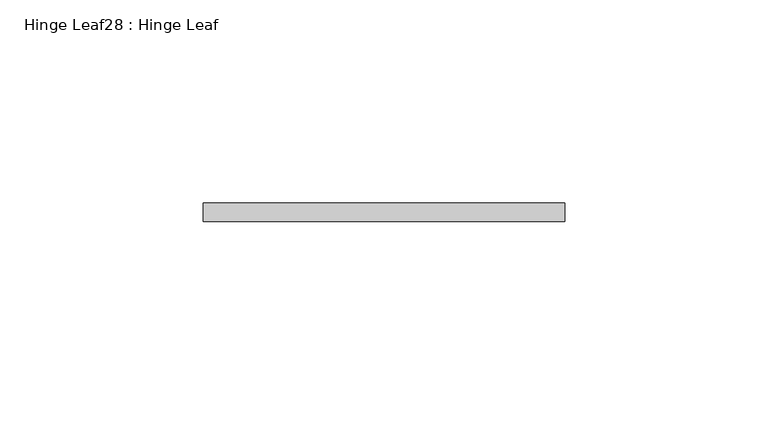
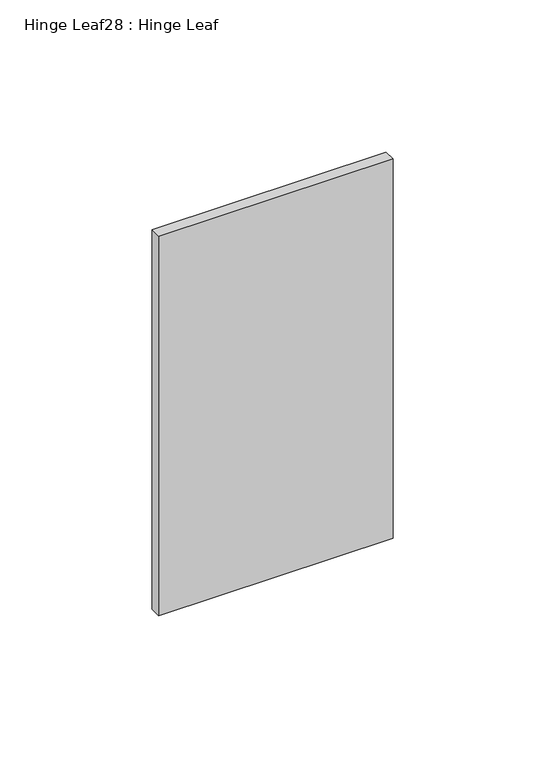
"""IFC4 building model written with IfcOpenShell, lengths in millimetres: proxy geometry, Hinge Leaf28 : Hinge Leaf."""

from ifc_helpers import new_model, si_unit, frame, origin, place, context, project, spatial, polyline, outline, extrude, source, transform, mapped, element, save


def hinge_leaf28_hinge_leaf_dc6140c5(model_context):
    return source(origin(), model_context, "Body", "SweptSolid", [
        extrude(outline(polyline([(587327.7934739, -531780.6943841), (587416.6934739, -531780.6943841), (587416.6934739, -531785.2663841), (587327.7934739, -531785.2663841), (587327.7934739, -531780.6943841)])), frame((0.0, 0.0, 1936.75), z_axis=(0.0, 0.0, 1.0), x_axis=(1.0, 0.0, 0.0)), (0.0, 0.0, 1.0), 152.4),
    ])


if __name__ == "__main__":
    model = new_model("IFC4")
    model_context = context("Model", 3, world=origin())
    ifc_project = project(units=[si_unit("LENGTHUNIT", "METRE", prefix="MILLI")], contexts=[model_context])
    site = spatial("IfcSite", under=ifc_project)
    building = spatial("IfcBuilding", under=site)
    placement = place(None, origin())
    hinge_leaf28_hinge_leaf_shape = hinge_leaf28_hinge_leaf_dc6140c5(model_context)
    element("IfcBuildingElementProxy", 1, Name="Hinge Leaf28 : Hinge Leaf", ObjectType="Hinge Leaf28 : Hinge Leaf", at=placement, inside=building, context=model_context, shape_type="MappedRepresentation", body=[
        mapped(hinge_leaf28_hinge_leaf_shape, transform((0.0, 0.0, 0.0), x_axis=(1.0, 0.0, 0.0), y_axis=(0.0, 1.0, 0.0), z_axis=(0.0, 0.0, 1.0))),
    ])
    save(model, "model.ifc")

# Revit data of these elements
# Element 1 (IfcBuildingElementProxy, "Hinge Leaf28 : Hinge Leaf")
#   Materials on its faces: "6\"X6\" WELD-ON STL BUTT HINGE"
# Materials
#   "6\"X6\" WELD-ON STL BUTT HINGE": class "Metal", colour RGB 189 187 185, transparency 0, Description = "Carbon steel", Cost = 0
